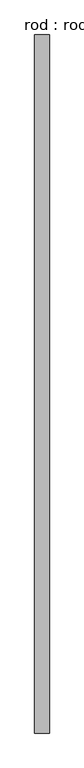
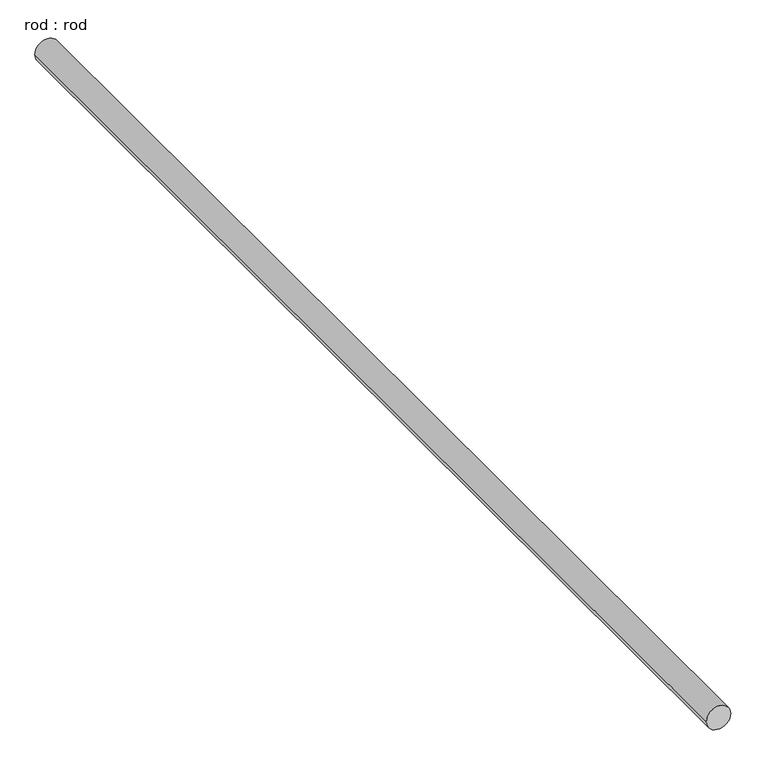
"""IFC4 building model written with IfcOpenShell, lengths in millimetres: proxy geometry, rod : rod."""

import ifcopenshell
import ifcopenshell.guid

model = None  # the IFC model being written
_history = None  # IfcOwnerHistory: only IFC2X3 demands one
_inside = {}  # id of a spatial element -> (the spatial element, [elements in it])
_under = {}  # id of a project, library or spatial element -> (it, [spatial elements below it])
_declared = {}  # id of a project -> (the project, [libraries it declares])
_typed = {}  # id of a type object -> (the type object, [elements of that type])
_made_of = {}  # id of a material, layer set ... -> (it, [elements and type objects made of it])


def new_model(schema):
    """Start an empty IFC model of exactly this schema.

    Asked for "IFC4X3", IfcOpenShell would pick the latest addendum, in which some entities
    have other attributes; the version numbers below select the first issue.
    IFC2X3 requires an IfcOwnerHistory on every rooted entity: one is made here for all.
    """
    global model, _history
    if schema == "IFC4X3":
        model = ifcopenshell.file(schema_version=(4, 3, 0, 0))
    else:
        model = ifcopenshell.file(schema=schema)
    _inside.clear()
    _under.clear()
    _declared.clear()
    _typed.clear()
    _made_of.clear()
    _history = None
    if model.schema == "IFC2X3":
        org = make("IfcOrganization", Name="unknown")
        user = make(
            "IfcPersonAndOrganization",
            ThePerson=make("IfcPerson", FamilyName="unknown"),
            TheOrganization=org,
        )
        app = make(
            "IfcApplication",
            ApplicationDeveloper=org,
            Version="unknown",
            ApplicationFullName="unknown",
            ApplicationIdentifier="unknown",
        )
        _history = make(
            "IfcOwnerHistory",
            OwningUser=user,
            OwningApplication=app,
            ChangeAction="ADDED",
            CreationDate=0,
        )
    return model


def make(cls, **values):
    """One entity of the class cls with the attributes given. An attribute that is None is left unset."""
    return model.create_entity(
        cls, **{name: value for name, value in values.items() if value is not None}
    )


def rooted(cls, **values):
    """An entity with a GlobalId (a new one), such as an element, a storey or a relation."""
    return make(cls, GlobalId=ifcopenshell.guid.new(), OwnerHistory=_history, **values)


def si_unit(unit_type, name, prefix=None):
    """IfcSIUnit, for example si_unit("LENGTHUNIT", "METRE", prefix="MILLI")."""
    return make("IfcSIUnit", UnitType=unit_type, Prefix=prefix, Name=name)


def assignment(units):
    """IfcUnitAssignment: the units of a project."""
    return None if units is None else make("IfcUnitAssignment", Units=units)


def point(xyz):
    """IfcCartesianPoint."""
    return None if xyz is None else make("IfcCartesianPoint", Coordinates=xyz)


def direction(xyz):
    """IfcDirection."""
    return None if xyz is None else make("IfcDirection", DirectionRatios=xyz)


def frame(location, z_axis=None, x_axis=None):
    """IfcAxis2Placement3D, a coordinate frame: its origin and axes. An axis left out is left unset."""
    return make(
        "IfcAxis2Placement3D",
        Location=point(location),
        Axis=direction(z_axis),
        RefDirection=direction(x_axis),
    )


def frame_2d(location, x_axis=None):
    """IfcAxis2Placement2D, a coordinate frame in the plane: its origin and x axis."""
    return make(
        "IfcAxis2Placement2D", Location=point(location), RefDirection=direction(x_axis)
    )


def origin():
    """The frame at (0, 0, 0) with its axes left unset."""
    return frame((0.0, 0.0, 0.0))


def place(relative_to, where):
    """IfcLocalPlacement: puts the frame where relative to a parent placement (None: the world)."""
    return make(
        "IfcLocalPlacement", PlacementRelTo=relative_to, RelativePlacement=where
    )


def context(
    kind, dimensions, precision=None, world=None, true_north=None, identifier=None
):
    """IfcGeometricRepresentationContext, for example the 3D "Model" context."""
    return make(
        "IfcGeometricRepresentationContext",
        ContextIdentifier=identifier,
        ContextType=kind,
        CoordinateSpaceDimension=dimensions,
        Precision=precision,
        WorldCoordinateSystem=world,
        TrueNorth=true_north,
    )


def project(units=None, contexts=None):
    """IfcProject with its units and contexts."""
    return rooted(
        "IfcProject",
        Name="project",
        RepresentationContexts=contexts,
        UnitsInContext=assignment(units),
    )


def spatial(cls, under=None, at=None, **own):
    """A site, building, storey or space (cls), placed at a placement, below another one or the project."""
    s = rooted(cls, ObjectPlacement=at, **own)
    if under is not None:
        _under.setdefault(under.id(), (under, []))[1].append(s)
    return s


def circle_curve(where, radius):
    """IfcCircle in the frame where."""
    return make("IfcCircle", Position=where, Radius=radius)


def trimmed(basis, trim1, trim2, sense, master):
    """IfcTrimmedCurve: the piece of a basis curve between two trims."""
    return make(
        "IfcTrimmedCurve",
        BasisCurve=basis,
        Trim1=trim1,
        Trim2=trim2,
        SenseAgreement=sense,
        MasterRepresentation=master,
    )


def segment(curve, same_sense, transition):
    """IfcCompositeCurveSegment."""
    return make(
        "IfcCompositeCurveSegment",
        Transition=transition,
        SameSense=same_sense,
        ParentCurve=curve,
    )


def composite_curve(segments, self_intersect=None):
    """IfcCompositeCurve: segments joined end to end."""
    return make("IfcCompositeCurve", Segments=segments, SelfIntersect=self_intersect)


def outline(outer, holes=None, kind="AREA"):
    """IfcArbitraryClosedProfileDef: a profile drawn as a closed curve; with holes, ...WithVoids."""
    if holes is None:
        return make("IfcArbitraryClosedProfileDef", ProfileType=kind, OuterCurve=outer)
    return make(
        "IfcArbitraryProfileDefWithVoids",
        ProfileType=kind,
        OuterCurve=outer,
        InnerCurves=holes,
    )


def extrude(swept, where, along, depth):
    """IfcExtrudedAreaSolid: the profile swept, set in the frame where, extruded along a direction by depth."""
    return make(
        "IfcExtrudedAreaSolid",
        SweptArea=swept,
        Position=where,
        ExtrudedDirection=direction(along),
        Depth=depth,
    )


def shape(context_of_items, identifier, shape_type, items):
    """IfcShapeRepresentation: the items that make up one representation, for example the "Body"."""
    return make(
        "IfcShapeRepresentation",
        ContextOfItems=context_of_items,
        RepresentationIdentifier=identifier,
        RepresentationType=shape_type,
        Items=items,
    )


def source(mapping_origin, context_of_items, identifier, shape_type, items):
    """IfcRepresentationMap: a shape defined once, which mapped items show again and again."""
    return make(
        "IfcRepresentationMap",
        MappingOrigin=mapping_origin,
        MappedRepresentation=shape(context_of_items, identifier, shape_type, items),
    )


def transform(
    local_origin,
    x_axis=None,
    y_axis=None,
    z_axis=None,
    scale=None,
    scale2=None,
    scale3=None,
    uniform=True,
):
    """IfcCartesianTransformationOperator3D, or its non-uniform kind. x_axis, y_axis, z_axis: its Axis1, 2, 3."""
    if uniform:
        return make(
            "IfcCartesianTransformationOperator3D",
            Axis1=direction(x_axis),
            Axis2=direction(y_axis),
            LocalOrigin=point(local_origin),
            Scale=scale,
            Axis3=direction(z_axis),
        )
    return make(
        "IfcCartesianTransformationOperator3DnonUniform",
        Axis1=direction(x_axis),
        Axis2=direction(y_axis),
        LocalOrigin=point(local_origin),
        Scale=scale,
        Axis3=direction(z_axis),
        Scale2=scale2,
        Scale3=scale3,
    )


def mapped(mapping_source, mapping_target):
    """IfcMappedItem: shows the shape of a source again, moved by a transform."""
    return make(
        "IfcMappedItem", MappingSource=mapping_source, MappingTarget=mapping_target
    )


def made_of(thing, what):
    """Note that an element or type object is made of a material, layer set ...; save() writes the relation."""
    if what is not None:
        _made_of.setdefault(what.id(), (what, []))[1].append(thing)
    return thing


def element(
    cls,
    number,
    at=None,
    inside=None,
    cuts=None,
    type_object=None,
    material=None,
    context=None,
    identifier="Body",
    shape_type=None,
    held_by="IfcProductDefinitionShape",
    body=None,
    shapes=None,
    **own,
):
    """One element of the class cls, such as IfcWall. Its Tag is "e" and its number.

    at: its placement. inside: the storey or other place that contains it. cuts: it is an
    opening in that element (IfcRelVoidsElement). A single representation is given by context,
    identifier, shape_type and body (its items); several are given by shapes. held_by: the class
    of the entity that holds the representations. save() writes the other relations.
    """
    e = rooted(cls, Tag="e%d" % number, ObjectPlacement=at, **own)
    if body is not None:
        shapes = [shape(context, identifier, shape_type, body)]
    if shapes is not None:
        e.Representation = make(held_by, Representations=shapes)
    if inside is not None:
        _inside.setdefault(inside.id(), (inside, []))[1].append(e)
    if cuts is not None:
        rooted(
            "IfcRelVoidsElement", RelatingBuildingElement=cuts, RelatedOpeningElement=e
        )
    if type_object is not None:
        _typed.setdefault(type_object.id(), (type_object, []))[1].append(e)
    return made_of(e, material)


def aggregate(whole, parts):
    """IfcRelAggregates: a whole, such as a stair, and the parts it consists of."""
    return rooted("IfcRelAggregates", RelatingObject=whole, RelatedObjects=parts)


def save(model, path):
    """Write the relations noted so far, then the file.

    IfcRelAggregates (storeys below a building ...), IfcRelContainedInSpatialStructure (elements
    in a storey), IfcRelDefinesByType, IfcRelAssociatesMaterial and IfcRelDeclares: one each for
    every whole, place, type object, material and project.
    """
    for whole, parts in _under.values():
        aggregate(whole, parts)
    for where, things in _inside.values():
        rooted(
            "IfcRelContainedInSpatialStructure",
            RelatedElements=things,
            RelatingStructure=where,
        )
    for kind, things in _typed.values():
        rooted("IfcRelDefinesByType", RelatedObjects=things, RelatingType=kind)
    for what, things in _made_of.values():
        rooted("IfcRelAssociatesMaterial", RelatedObjects=things, RelatingMaterial=what)
    for by, libraries in _declared.values():
        rooted("IfcRelDeclares", RelatingContext=by, RelatedDefinitions=libraries)
    model.write(path)


def rod_rod_95733b82(model_context):
    return source(origin(), model_context, "Body", "SweptSolid", [
        extrude(outline(composite_curve([segment(trimmed(circle_curve(frame_2d((0.0108462, 0.0)), 200.0), [point((0.0108462, 200.0))], [point((0.0108462, -200.0))], False, "CARTESIAN"), True, "CONTINUOUS"), segment(trimmed(circle_curve(frame_2d((0.0108462, 0.0)), 200.0), [point((0.0108462, -200.0))], [point((0.0108462, 200.0))], False, "CARTESIAN"), True, "CONTINUOUS")], self_intersect=False)), frame((0.0, -5444.8942541, 0.0), z_axis=(0.0, 1.0, 0.0), x_axis=(0.0, 0.0, 1.0)), (0.0, 0.0, 1.0), 19075.2457389),
    ])


if __name__ == "__main__":
    model = new_model("IFC4")
    model_context = context("Model", 3, world=origin())
    ifc_project = project(units=[si_unit("LENGTHUNIT", "METRE", prefix="MILLI")], contexts=[model_context])
    site = spatial("IfcSite", under=ifc_project)
    building = spatial("IfcBuilding", under=site)
    placement = place(None, origin())
    rod_rod_shape = rod_rod_95733b82(model_context)
    element("IfcBuildingElementProxy", 1, Name="rod : rod", ObjectType="rod : rod", at=placement, inside=building, context=model_context, shape_type="MappedRepresentation", body=[
        mapped(rod_rod_shape, transform((0.0, 0.0, 0.0), x_axis=(1.0, 0.0, 0.0), y_axis=(0.0, 1.0, 0.0), z_axis=(0.0, 0.0, 1.0))),
    ])
    save(model, "model.ifc")

# Revit data of these elements
# Type "rod : rod"
#   Default Elevation = 0
